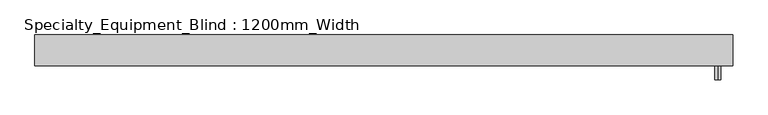
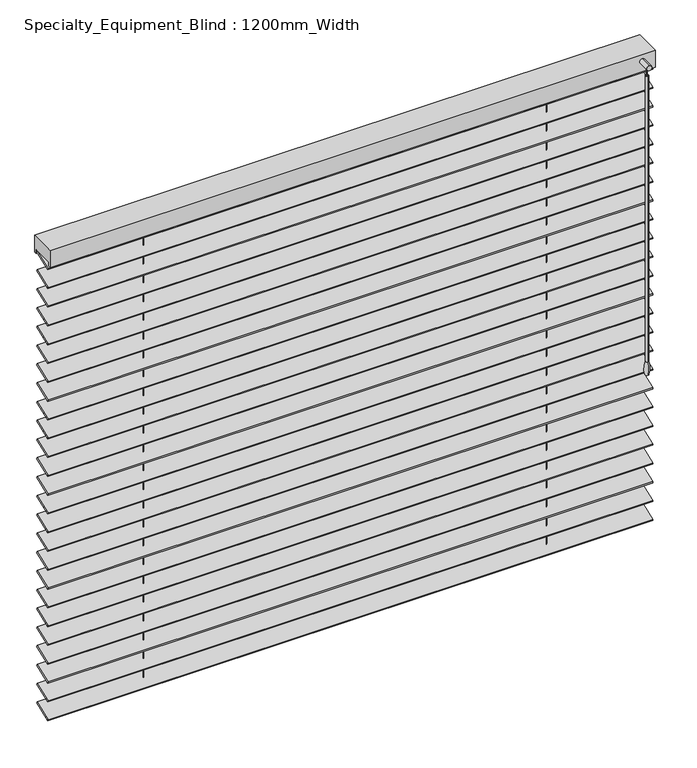
"""IFC4 building model written with IfcOpenShell, lengths in millimetres: proxy geometry, Specialty_Equipment_Blind : 1200mm_Width."""

import ifcopenshell
import ifcopenshell.guid

model = None  # the IFC model being written
_history = None  # IfcOwnerHistory: only IFC2X3 demands one
_inside = {}  # id of a spatial element -> (the spatial element, [elements in it])
_under = {}  # id of a project, library or spatial element -> (it, [spatial elements below it])
_declared = {}  # id of a project -> (the project, [libraries it declares])
_typed = {}  # id of a type object -> (the type object, [elements of that type])
_made_of = {}  # id of a material, layer set ... -> (it, [elements and type objects made of it])


def new_model(schema):
    """Start an empty IFC model of exactly this schema.

    Asked for "IFC4X3", IfcOpenShell would pick the latest addendum, in which some entities
    have other attributes; the version numbers below select the first issue.
    IFC2X3 requires an IfcOwnerHistory on every rooted entity: one is made here for all.
    """
    global model, _history
    if schema == "IFC4X3":
        model = ifcopenshell.file(schema_version=(4, 3, 0, 0))
    else:
        model = ifcopenshell.file(schema=schema)
    _inside.clear()
    _under.clear()
    _declared.clear()
    _typed.clear()
    _made_of.clear()
    _history = None
    if model.schema == "IFC2X3":
        org = make("IfcOrganization", Name="unknown")
        user = make(
            "IfcPersonAndOrganization",
            ThePerson=make("IfcPerson", FamilyName="unknown"),
            TheOrganization=org,
        )
        app = make(
            "IfcApplication",
            ApplicationDeveloper=org,
            Version="unknown",
            ApplicationFullName="unknown",
            ApplicationIdentifier="unknown",
        )
        _history = make(
            "IfcOwnerHistory",
            OwningUser=user,
            OwningApplication=app,
            ChangeAction="ADDED",
            CreationDate=0,
        )
    return model


def make(cls, **values):
    """One entity of the class cls with the attributes given. An attribute that is None is left unset."""
    return model.create_entity(
        cls, **{name: value for name, value in values.items() if value is not None}
    )


def rooted(cls, **values):
    """An entity with a GlobalId (a new one), such as an element, a storey or a relation."""
    return make(cls, GlobalId=ifcopenshell.guid.new(), OwnerHistory=_history, **values)


def si_unit(unit_type, name, prefix=None):
    """IfcSIUnit, for example si_unit("LENGTHUNIT", "METRE", prefix="MILLI")."""
    return make("IfcSIUnit", UnitType=unit_type, Prefix=prefix, Name=name)


def assignment(units):
    """IfcUnitAssignment: the units of a project."""
    return None if units is None else make("IfcUnitAssignment", Units=units)


def point(xyz):
    """IfcCartesianPoint."""
    return None if xyz is None else make("IfcCartesianPoint", Coordinates=xyz)


def direction(xyz):
    """IfcDirection."""
    return None if xyz is None else make("IfcDirection", DirectionRatios=xyz)


def frame(location, z_axis=None, x_axis=None):
    """IfcAxis2Placement3D, a coordinate frame: its origin and axes. An axis left out is left unset."""
    return make(
        "IfcAxis2Placement3D",
        Location=point(location),
        Axis=direction(z_axis),
        RefDirection=direction(x_axis),
    )


def frame_2d(location, x_axis=None):
    """IfcAxis2Placement2D, a coordinate frame in the plane: its origin and x axis."""
    return make(
        "IfcAxis2Placement2D", Location=point(location), RefDirection=direction(x_axis)
    )


def origin():
    """The frame at (0, 0, 0) with its axes left unset."""
    return frame((0.0, 0.0, 0.0))


def place(relative_to, where):
    """IfcLocalPlacement: puts the frame where relative to a parent placement (None: the world)."""
    return make(
        "IfcLocalPlacement", PlacementRelTo=relative_to, RelativePlacement=where
    )


def context(
    kind, dimensions, precision=None, world=None, true_north=None, identifier=None
):
    """IfcGeometricRepresentationContext, for example the 3D "Model" context."""
    return make(
        "IfcGeometricRepresentationContext",
        ContextIdentifier=identifier,
        ContextType=kind,
        CoordinateSpaceDimension=dimensions,
        Precision=precision,
        WorldCoordinateSystem=world,
        TrueNorth=true_north,
    )


def project(units=None, contexts=None):
    """IfcProject with its units and contexts."""
    return rooted(
        "IfcProject",
        Name="project",
        RepresentationContexts=contexts,
        UnitsInContext=assignment(units),
    )


def spatial(cls, under=None, at=None, **own):
    """A site, building, storey or space (cls), placed at a placement, below another one or the project."""
    s = rooted(cls, ObjectPlacement=at, **own)
    if under is not None:
        _under.setdefault(under.id(), (under, []))[1].append(s)
    return s


def polyline(points):
    """IfcPolyline through the points."""
    return make("IfcPolyline", Points=[point(p) for p in points])


def circle_curve(where, radius):
    """IfcCircle in the frame where."""
    return make("IfcCircle", Position=where, Radius=radius)


def ellipse_curve(where, semi_axis1, semi_axis2):
    """IfcEllipse in the frame where."""
    return make(
        "IfcEllipse", Position=where, SemiAxis1=semi_axis1, SemiAxis2=semi_axis2
    )


def trimmed(basis, trim1, trim2, sense, master):
    """IfcTrimmedCurve: the piece of a basis curve between two trims."""
    return make(
        "IfcTrimmedCurve",
        BasisCurve=basis,
        Trim1=trim1,
        Trim2=trim2,
        SenseAgreement=sense,
        MasterRepresentation=master,
    )


def segment(curve, same_sense, transition):
    """IfcCompositeCurveSegment."""
    return make(
        "IfcCompositeCurveSegment",
        Transition=transition,
        SameSense=same_sense,
        ParentCurve=curve,
    )


def composite_curve(segments, self_intersect=None):
    """IfcCompositeCurve: segments joined end to end."""
    return make("IfcCompositeCurve", Segments=segments, SelfIntersect=self_intersect)


def outline(outer, holes=None, kind="AREA"):
    """IfcArbitraryClosedProfileDef: a profile drawn as a closed curve; with holes, ...WithVoids."""
    if holes is None:
        return make("IfcArbitraryClosedProfileDef", ProfileType=kind, OuterCurve=outer)
    return make(
        "IfcArbitraryProfileDefWithVoids",
        ProfileType=kind,
        OuterCurve=outer,
        InnerCurves=holes,
    )


def extrude(swept, where, along, depth):
    """IfcExtrudedAreaSolid: the profile swept, set in the frame where, extruded along a direction by depth."""
    return make(
        "IfcExtrudedAreaSolid",
        SweptArea=swept,
        Position=where,
        ExtrudedDirection=direction(along),
        Depth=depth,
    )


def shape(context_of_items, identifier, shape_type, items):
    """IfcShapeRepresentation: the items that make up one representation, for example the "Body"."""
    return make(
        "IfcShapeRepresentation",
        ContextOfItems=context_of_items,
        RepresentationIdentifier=identifier,
        RepresentationType=shape_type,
        Items=items,
    )


def source(mapping_origin, context_of_items, identifier, shape_type, items):
    """IfcRepresentationMap: a shape defined once, which mapped items show again and again."""
    return make(
        "IfcRepresentationMap",
        MappingOrigin=mapping_origin,
        MappedRepresentation=shape(context_of_items, identifier, shape_type, items),
    )


def transform(
    local_origin,
    x_axis=None,
    y_axis=None,
    z_axis=None,
    scale=None,
    scale2=None,
    scale3=None,
    uniform=True,
):
    """IfcCartesianTransformationOperator3D, or its non-uniform kind. x_axis, y_axis, z_axis: its Axis1, 2, 3."""
    if uniform:
        return make(
            "IfcCartesianTransformationOperator3D",
            Axis1=direction(x_axis),
            Axis2=direction(y_axis),
            LocalOrigin=point(local_origin),
            Scale=scale,
            Axis3=direction(z_axis),
        )
    return make(
        "IfcCartesianTransformationOperator3DnonUniform",
        Axis1=direction(x_axis),
        Axis2=direction(y_axis),
        LocalOrigin=point(local_origin),
        Scale=scale,
        Axis3=direction(z_axis),
        Scale2=scale2,
        Scale3=scale3,
    )


def mapped(mapping_source, mapping_target):
    """IfcMappedItem: shows the shape of a source again, moved by a transform."""
    return make(
        "IfcMappedItem", MappingSource=mapping_source, MappingTarget=mapping_target
    )


def made_of(thing, what):
    """Note that an element or type object is made of a material, layer set ...; save() writes the relation."""
    if what is not None:
        _made_of.setdefault(what.id(), (what, []))[1].append(thing)
    return thing


def element(
    cls,
    number,
    at=None,
    inside=None,
    cuts=None,
    type_object=None,
    material=None,
    context=None,
    identifier="Body",
    shape_type=None,
    held_by="IfcProductDefinitionShape",
    body=None,
    shapes=None,
    **own,
):
    """One element of the class cls, such as IfcWall. Its Tag is "e" and its number.

    at: its placement. inside: the storey or other place that contains it. cuts: it is an
    opening in that element (IfcRelVoidsElement). A single representation is given by context,
    identifier, shape_type and body (its items); several are given by shapes. held_by: the class
    of the entity that holds the representations. save() writes the other relations.
    """
    e = rooted(cls, Tag="e%d" % number, ObjectPlacement=at, **own)
    if body is not None:
        shapes = [shape(context, identifier, shape_type, body)]
    if shapes is not None:
        e.Representation = make(held_by, Representations=shapes)
    if inside is not None:
        _inside.setdefault(inside.id(), (inside, []))[1].append(e)
    if cuts is not None:
        rooted(
            "IfcRelVoidsElement", RelatingBuildingElement=cuts, RelatedOpeningElement=e
        )
    if type_object is not None:
        _typed.setdefault(type_object.id(), (type_object, []))[1].append(e)
    return made_of(e, material)


def aggregate(whole, parts):
    """IfcRelAggregates: a whole, such as a stair, and the parts it consists of."""
    return rooted("IfcRelAggregates", RelatingObject=whole, RelatedObjects=parts)


def save(model, path):
    """Write the relations noted so far, then the file.

    IfcRelAggregates (storeys below a building ...), IfcRelContainedInSpatialStructure (elements
    in a storey), IfcRelDefinesByType, IfcRelAssociatesMaterial and IfcRelDeclares: one each for
    every whole, place, type object, material and project.
    """
    for whole, parts in _under.values():
        aggregate(whole, parts)
    for where, things in _inside.values():
        rooted(
            "IfcRelContainedInSpatialStructure",
            RelatedElements=things,
            RelatingStructure=where,
        )
    for kind, things in _typed.values():
        rooted("IfcRelDefinesByType", RelatedObjects=things, RelatingType=kind)
    for what, things in _made_of.values():
        rooted("IfcRelAssociatesMaterial", RelatedObjects=things, RelatingMaterial=what)
    for by, libraries in _declared.values():
        rooted("IfcRelDeclares", RelatingContext=by, RelatedDefinitions=libraries)
    model.write(path)


def plane_surface(at):
    """IfcPlane: the flat surface through the origin of the frame at, square to its z axis."""
    return make("IfcPlane", Position=at)


def cylinder_surface(at, radius):
    """IfcCylindricalSurface: all points at the distance radius from the z axis of the frame at."""
    return make("IfcCylindricalSurface", Position=at, Radius=radius)


def revolved_surface(curve, axis_point, axis_direction):
    """IfcSurfaceOfRevolution: the curve turned about the line through axis_point along axis_direction."""
    return make(
        "IfcSurfaceOfRevolution",
        SweptCurve=make("IfcArbitraryOpenProfileDef", ProfileType="CURVE", Curve=curve),
        AxisPosition=make("IfcAxis1Placement", Location=point(axis_point), Axis=direction(axis_direction)),
    )


def advanced_brep(points, edges, surfaces, faces):
    """IfcAdvancedBrep: a solid bounded by faces that lie on surfaces and meet in shared edges.

    An edge is (start, end): straight between two places in points (the first is 0);
    or (start, end, curve); or (start, end, curve, False) where it runs against its curve.
    A face is (place in surfaces, loops), or (place, loops, False) where it looks against
    its surface's normal. A loop lists edges by number (the first is 1), with a minus sign
    where the edge is run from its end to its start. The first loop is the outer one.
    """
    corners = [point(p) for p in points]
    vertices = [make("IfcVertexPoint", VertexGeometry=c) for c in corners]
    made = []
    for start, end, *more in edges:
        made.append(
            make(
                "IfcEdgeCurve",
                EdgeStart=vertices[start],
                EdgeEnd=vertices[end],
                EdgeGeometry=more[0] if more else make("IfcPolyline", Points=[corners[start], corners[end]]),
                SameSense=more[1] if len(more) > 1 else True,
            )
        )
    hull = []
    for where, loops, *sense in faces:
        bounds = []
        for j, loop in enumerate(loops):
            ring = [make("IfcOrientedEdge", EdgeElement=made[abs(k) - 1], Orientation=k > 0) for k in loop]
            bounds.append(
                make(
                    "IfcFaceOuterBound" if j == 0 else "IfcFaceBound",
                    Bound=make("IfcEdgeLoop", EdgeList=ring),
                    Orientation=True,
                )
            )
        hull.append(make("IfcAdvancedFace", Bounds=bounds, FaceSurface=surfaces[where], SameSense=sense[0] if sense else True))
    return make("IfcAdvancedBrep", Outer=make("IfcClosedShell", CfsFaces=hull))


def specialty_equipment_blind_1200mm_width_23c077ca(model_context):
    return source(origin(), model_context, "Body", "SolidModel", [
        extrude(outline(polyline([(0.0, -40.0), (0.0, 0.0), (1180.0, 0.0), (1180.0, -40.0), (0.0, -40.0)])), frame((-439.5079376, 65.0532351, 2040.2125618), z_axis=(0.0, -0.3420201433256684, 0.9396926207859085), x_axis=(1.0, 0.0, 0.0)), (0.0, 0.0, 1.0), 3.0625345),
        extrude(outline(polyline([(0.0, -40.0), (0.0, 0.0), (1180.0, 0.0), (1180.0, -40.0), (0.0, -40.0)])), frame((-439.5079376, 65.0532351, 2001.4625618), z_axis=(0.0, -0.3420201433256684, 0.9396926207859085), x_axis=(1.0, 0.0, 0.0)), (0.0, 0.0, 1.0), 3.0625345),
        extrude(outline(polyline([(0.0, -40.0), (0.0, 0.0), (1180.0, 0.0), (1180.0, -40.0), (0.0, -40.0)])), frame((-439.5079376, 65.0532351, 1962.7125618), z_axis=(0.0, -0.3420201433256684, 0.9396926207859085), x_axis=(1.0, 0.0, 0.0)), (0.0, 0.0, 1.0), 3.0625345),
        extrude(outline(polyline([(0.0, -40.0), (0.0, 0.0), (1180.0, 0.0), (1180.0, -40.0), (0.0, -40.0)])), frame((-439.5079376, 65.0532351, 1923.9625618), z_axis=(0.0, -0.3420201433256684, 0.9396926207859085), x_axis=(1.0, 0.0, 0.0)), (0.0, 0.0, 1.0), 3.0625345),
        extrude(outline(polyline([(0.0, -40.0), (0.0, 0.0), (1180.0, 0.0), (1180.0, -40.0), (0.0, -40.0)])), frame((-439.5079376, 65.0532351, 1885.2125618), z_axis=(0.0, -0.3420201433256684, 0.9396926207859085), x_axis=(1.0, 0.0, 0.0)), (0.0, 0.0, 1.0), 3.0625345),
        extrude(outline(polyline([(0.0, -40.0), (0.0, 0.0), (1180.0, 0.0), (1180.0, -40.0), (0.0, -40.0)])), frame((-439.5079376, 65.0532351, 1846.4625618), z_axis=(0.0, -0.3420201433256684, 0.9396926207859085), x_axis=(1.0, 0.0, 0.0)), (0.0, 0.0, 1.0), 3.0625345),
        extrude(outline(polyline([(0.0, -40.0), (0.0, 0.0), (1180.0, 0.0), (1180.0, -40.0), (0.0, -40.0)])), frame((-439.5079376, 65.0532351, 1807.7125618), z_axis=(0.0, -0.3420201433256684, 0.9396926207859085), x_axis=(1.0, 0.0, 0.0)), (0.0, 0.0, 1.0), 3.0625345),
        extrude(outline(polyline([(0.0, -40.0), (0.0, 0.0), (1180.0, 0.0), (1180.0, -40.0), (0.0, -40.0)])), frame((-439.5079376, 65.0532351, 1768.9625618), z_axis=(0.0, -0.3420201433256684, 0.9396926207859085), x_axis=(1.0, 0.0, 0.0)), (0.0, 0.0, 1.0), 3.0625345),
        extrude(outline(polyline([(0.0, -40.0), (0.0, 0.0), (1180.0, 0.0), (1180.0, -40.0), (0.0, -40.0)])), frame((-439.5079376, 65.0532351, 1730.2125618), z_axis=(0.0, -0.3420201433256684, 0.9396926207859085), x_axis=(1.0, 0.0, 0.0)), (0.0, 0.0, 1.0), 3.0625345),
        extrude(outline(polyline([(0.0, -40.0), (0.0, 0.0), (1180.0, 0.0), (1180.0, -40.0), (0.0, -40.0)])), frame((-439.5079376, 65.0532351, 1691.4625618), z_axis=(0.0, -0.3420201433256684, 0.9396926207859085), x_axis=(1.0, 0.0, 0.0)), (0.0, 0.0, 1.0), 3.0625345),
        extrude(outline(polyline([(0.0, -40.0), (0.0, 0.0), (1180.0, 0.0), (1180.0, -40.0), (0.0, -40.0)])), frame((-439.5079376, 65.0532351, 1652.7125618), z_axis=(0.0, -0.3420201433256684, 0.9396926207859085), x_axis=(1.0, 0.0, 0.0)), (0.0, 0.0, 1.0), 3.0625345),
        extrude(outline(polyline([(0.0, -40.0), (0.0, 0.0), (1180.0, 0.0), (1180.0, -40.0), (0.0, -40.0)])), frame((-439.5079376, 65.0532351, 1613.9625618), z_axis=(0.0, -0.3420201433256684, 0.9396926207859085), x_axis=(1.0, 0.0, 0.0)), (0.0, 0.0, 1.0), 3.0625345),
        extrude(outline(polyline([(0.0, -40.0), (0.0, 0.0), (1180.0, 0.0), (1180.0, -40.0), (0.0, -40.0)])), frame((-439.5079376, 65.0532351, 1575.2125618), z_axis=(0.0, -0.3420201433256684, 0.9396926207859085), x_axis=(1.0, 0.0, 0.0)), (0.0, 0.0, 1.0), 3.0625345),
        extrude(outline(polyline([(0.0, -40.0), (0.0, 0.0), (1180.0, 0.0), (1180.0, -40.0), (0.0, -40.0)])), frame((-439.5079376, 65.0532351, 1536.4625618), z_axis=(0.0, -0.3420201433256684, 0.9396926207859085), x_axis=(1.0, 0.0, 0.0)), (0.0, 0.0, 1.0), 3.0625345),
        extrude(outline(polyline([(0.0, -40.0), (0.0, 0.0), (1180.0, 0.0), (1180.0, -40.0), (0.0, -40.0)])), frame((-439.5079376, 65.0532351, 1497.7125618), z_axis=(0.0, -0.3420201433256684, 0.9396926207859085), x_axis=(1.0, 0.0, 0.0)), (0.0, 0.0, 1.0), 3.0625345),
        extrude(outline(polyline([(0.0, -40.0), (0.0, 0.0), (1180.0, 0.0), (1180.0, -40.0), (0.0, -40.0)])), frame((-439.5079376, 65.0532351, 1458.9625618), z_axis=(0.0, -0.3420201433256684, 0.9396926207859085), x_axis=(1.0, 0.0, 0.0)), (0.0, 0.0, 1.0), 3.0625345),
        extrude(outline(polyline([(0.0, -40.0), (0.0, 0.0), (1180.0, 0.0), (1180.0, -40.0), (0.0, -40.0)])), frame((-439.5079376, 65.0532351, 1420.2125618), z_axis=(0.0, -0.3420201433256684, 0.9396926207859085), x_axis=(1.0, 0.0, 0.0)), (0.0, 0.0, 1.0), 3.0625345),
        extrude(outline(polyline([(0.0, -40.0), (0.0, 0.0), (1180.0, 0.0), (1180.0, -40.0), (0.0, -40.0)])), frame((-439.5079376, 65.0532351, 1381.4625618), z_axis=(0.0, -0.3420201433256684, 0.9396926207859085), x_axis=(1.0, 0.0, 0.0)), (0.0, 0.0, 1.0), 3.0625345),
        extrude(outline(polyline([(0.0, -40.0), (0.0, 0.0), (1180.0, 0.0), (1180.0, -40.0), (0.0, -40.0)])), frame((-439.5079376, 65.0532351, 1342.7125618), z_axis=(0.0, -0.3420201433256684, 0.9396926207859085), x_axis=(1.0, 0.0, 0.0)), (0.0, 0.0, 1.0), 3.0625345),
        extrude(outline(polyline([(0.0, -40.0), (0.0, 0.0), (1180.0, 0.0), (1180.0, -40.0), (0.0, -40.0)])), frame((-439.5079376, 65.0532351, 1303.9625618), z_axis=(0.0, -0.3420201433256684, 0.9396926207859085), x_axis=(1.0, 0.0, 0.0)), (0.0, 0.0, 1.0), 3.0625345),
        extrude(outline(polyline([(0.0, -40.0), (0.0, 0.0), (1180.0, 0.0), (1180.0, -40.0), (0.0, -40.0)])), frame((-439.5079376, 65.0532351, 1265.2125618), z_axis=(0.0, -0.3420201433256684, 0.9396926207859085), x_axis=(1.0, 0.0, 0.0)), (0.0, 0.0, 1.0), 3.0625345),
        extrude(outline(polyline([(0.0, -40.0), (0.0, 0.0), (1180.0, 0.0), (1180.0, -40.0), (0.0, -40.0)])), frame((-439.5079376, 65.0532351, 1226.4625618), z_axis=(0.0, -0.3420201433256684, 0.9396926207859085), x_axis=(1.0, 0.0, 0.0)), (0.0, 0.0, 1.0), 3.0625345),
        extrude(outline(polyline([(0.0, -40.0), (0.0, 0.0), (1180.0, 0.0), (1180.0, -40.0), (0.0, -40.0)])), frame((-439.5079376, 65.0532351, 1187.7125618), z_axis=(0.0, -0.3420201433256684, 0.9396926207859085), x_axis=(1.0, 0.0, 0.0)), (0.0, 0.0, 1.0), 3.0625345),
        extrude(outline(polyline([(0.0, -40.0), (0.0, 0.0), (1180.0, 0.0), (1180.0, -40.0), (0.0, -40.0)])), frame((-439.5079376, 65.0532351, 2078.9625618), z_axis=(0.0, -0.3420201433256684, 0.9396926207859085), x_axis=(1.0, 0.0, 0.0)), (0.0, 0.0, 1.0), 3.0625345),
        extrude(outline(polyline([(0.0, -40.0), (0.0, 0.0), (1180.0, 0.0), (1180.0, -40.0), (0.0, -40.0)])), frame((-439.5079376, 65.0532351, 1148.9625618), z_axis=(0.0, -0.3420201433256684, 0.9396926207859085), x_axis=(1.0, 0.0, 0.0)), (0.0, 0.0, 1.0), 3.0625345),
        extrude(outline(composite_curve([segment(trimmed(circle_curve(frame_2d((-242.8412709, 45.2119342)), 0.5), [point((-243.3412709, 45.2119342))], [point((-242.3412709, 45.2119342))], False, "CARTESIAN"), True, "CONTINUOUS"), segment(trimmed(circle_curve(frame_2d((-242.8412709, 45.2119342)), 0.5), [point((-242.3412709, 45.2119342))], [point((-243.3412709, 45.2119342))], False, "CARTESIAN"), True, "CONTINUOUS")], self_intersect=False)), frame((0.0, 0.0, 1130.0), z_axis=(0.0, 0.0, 1.0), x_axis=(1.0, 0.0, 0.0)), (0.0, 0.0, 1.0), 953.2448883),
        extrude(outline(composite_curve([segment(trimmed(circle_curve(frame_2d((543.8253958, 45.2119342)), 0.5), [point((543.3253958, 45.2119342))], [point((544.3253958, 45.2119342))], False, "CARTESIAN"), True, "CONTINUOUS"), segment(trimmed(circle_curve(frame_2d((543.8253958, 45.2119342)), 0.5), [point((544.3253958, 45.2119342))], [point((543.3253958, 45.2119342))], False, "CARTESIAN"), True, "CONTINUOUS")], self_intersect=False)), frame((0.0, 0.0, 1130.0), z_axis=(0.0, 0.0, 1.0), x_axis=(1.0, 0.0, 0.0)), (0.0, 0.0, 1.0), 953.2448883),
        advanced_brep(
        [(715.4920624, 4.7248495, 2091.3243671), (715.4920624, 2.7248495, 2091.3243671), (715.4920624, 3.7248495, 2091.3243671), (715.4920624, 4.7248495, 2076.3243671), (715.4920624, 2.7248495, 2076.3243671), (715.4920624, 6.7248495, 2076.3243671), (715.4920624, 0.7248495, 2076.3243671), (715.4920624, 6.7248495, 1486.909931), (715.4920624, 0.7248495, 1486.909931), (715.4920624, 7.2513368, 1460.0), (715.4920624, 0.1983622, 1460.0), (715.4920624, 3.7248495, 1460.0)],
        [
            (0, 1, circle_curve(frame((715.4920624, 3.7248495, 2091.3243671), z_axis=(0.0, 0.0, 1.0), x_axis=(0.0, -1.0, 0.0)), 1.0)),
            (1, 2),
            (2, 0),
            (1, 0, circle_curve(frame((715.4920624, 3.7248495, 2091.3243671), z_axis=(0.0, 0.0, 1.0), x_axis=(0.0, -1.0, 0.0)), 1.0)),
            (3, 4, circle_curve(frame((715.4920624, 3.7248495, 2076.3243671), z_axis=(0.0, 0.0, 1.0), x_axis=(0.0, -1.0, 0.0)), 1.0)),
            (4, 1),
            (0, 3),
            (4, 3, circle_curve(frame((715.4920624, 3.7248495, 2076.3243671), z_axis=(0.0, 0.0, 1.0), x_axis=(0.0, -1.0, 0.0)), 1.0)),
            (5, 6, circle_curve(frame((715.4920624, 3.7248495, 2076.3243671), z_axis=(0.0, 0.0, 1.0), x_axis=(0.0, -1.0, 0.0)), 3.0)),
            (6, 4),
            (3, 5),
            (6, 5, circle_curve(frame((715.4920624, 3.7248495, 2076.3243671), z_axis=(0.0, 0.0, 1.0), x_axis=(0.0, -1.0, 0.0)), 3.0)),
            (7, 8, circle_curve(frame((715.4920624, 3.7248495, 1486.909931), z_axis=(0.0, 0.0, 1.0), x_axis=(0.0, -1.0, 0.0)), 3.0)),
            (8, 6),
            (5, 7),
            (8, 7, circle_curve(frame((715.4920624, 3.7248495, 1486.909931), z_axis=(0.0, 0.0, 1.0), x_axis=(0.0, -1.0, 0.0)), 3.0)),
            (9, 10, circle_curve(frame((715.4920624, 3.7248495, 1460.0), z_axis=(0.0, 0.0, 1.0), x_axis=(0.0, -1.0, 0.0)), 3.5264873)),
            (10, 8, circle_curve(frame((715.4920624, 49.2720063, 1472.5), z_axis=(-1.0, 0.0, 0.0), x_axis=(0.0, 1.0, 0.0)), 50.6406214)),
            (7, 9, circle_curve(frame((715.4920624, -41.8223072, 1472.5), z_axis=(-1.0, 0.0, 0.0), x_axis=(0.0, -1.0, 0.0)), 50.6406214)),
            (10, 9, circle_curve(frame((715.4920624, 3.7248495, 1460.0), z_axis=(0.0, 0.0, 1.0), x_axis=(0.0, -1.0, 0.0)), 3.5264873)),
            (11, 10),
            (9, 11),
        ],
        [
            plane_surface(frame((715.4920624, 3.7248495, 2091.3243671), z_axis=(0.0, 0.0, 1.0), x_axis=(0.0, -1.0, 0.0))),
            cylinder_surface(frame((715.4920624, 3.7248495, 1191.3243671), z_axis=(0.0, 0.0, -1.0), x_axis=(0.0, -1.0, 0.0)), 1.0),
            plane_surface(frame((715.4920624, 3.7248495, 2076.3243671), z_axis=(0.0, 0.0, 1.0), x_axis=(0.0, -1.0, 0.0))),
            cylinder_surface(frame((715.4920624, 3.7248495, 1191.3243671), z_axis=(0.0, 0.0, -1.0), x_axis=(0.0, -1.0, 0.0)), 3.0),
            revolved_surface(trimmed(ellipse_curve(frame((715.4920624, 49.2720063, 1472.5), z_axis=(1.0, 0.0, 0.0), x_axis=(0.0, 1.0, 0.0)), 50.6406214, 50.6406214), [point((715.4920624, 0.7248495, 1486.909931))], [point((715.4920624, 0.1983622, 1460.0))], True, "CARTESIAN"), (715.4920624, 3.7248495, 1191.3243671), (0.0, 0.0, -1.0)),
            plane_surface(frame((715.4920624, 3.7248495, 1460.0), z_axis=(0.0, 0.0, -1.0), x_axis=(0.0, -1.0, 0.0))),
        ],
        [
            (0, [[1, 2, 3]]),
            (0, [[4, -3, -2]]),
            (1, [[5, 6, -1, 7]]),
            (1, [[8, -7, -4, -6]]),
            (2, [[9, 10, -5, 11]]),
            (2, [[12, -11, -8, -10]]),
            (3, [[13, 14, -9, 15]]),
            (3, [[16, -15, -12, -14]]),
            (4, [[17, 18, -13, 19]]),
            (4, [[20, -19, -16, -18]]),
            (5, [[21, -17, 22]]),
            (5, [[-22, -20, -21]]),
        ],
    ),
        extrude(outline(composite_curve([segment(trimmed(circle_curve(frame_2d((2095.9171213, 715.4920624)), 5.0), [point((2100.9171213, 715.4920624))], [point((2090.9171213, 715.4920624))], False, "CARTESIAN"), True, "CONTINUOUS"), segment(trimmed(circle_curve(frame_2d((2095.9171213, 715.4920624)), 5.0), [point((2090.9171213, 715.4920624))], [point((2100.9171213, 715.4920624))], False, "CARTESIAN"), True, "CONTINUOUS")], self_intersect=False)), frame((0.0, -4.4512463, 0.0), z_axis=(0.0, 1.0, 0.0), x_axis=(0.0, 0.0, 1.0)), (0.0, 0.0, 1.0), 23.7809602),
        extrude(outline(polyline([(19.329714, 2110.0), (71.0941545, 2110.0), (71.0941545, 2075.0), (66.0941545, 2075.0), (66.0941545, 2083.2448883), (24.329714, 2083.2448883), (24.329714, 2075.0), (19.329714, 2075.0), (19.329714, 2110.0)])), frame((-439.5079376, 0.0, 0.0), z_axis=(1.0, 0.0, 0.0), x_axis=(0.0, 1.0, 0.0)), (0.0, 0.0, 1.0), 1180.0),
    ])


if __name__ == "__main__":
    model = new_model("IFC4")
    model_context = context("Model", 3, world=origin())
    ifc_project = project(units=[si_unit("LENGTHUNIT", "METRE", prefix="MILLI")], contexts=[model_context])
    site = spatial("IfcSite", under=ifc_project)
    building = spatial("IfcBuilding", under=site)
    placement = place(None, origin())
    specialty_equipment_blind_1200mm_width_shape = specialty_equipment_blind_1200mm_width_23c077ca(model_context)
    element("IfcBuildingElementProxy", 1, Name="Specialty_Equipment_Blind : 1200mm_Width", ObjectType="Specialty_Equipment_Blind : 1200mm_Width", at=placement, inside=building, context=model_context, shape_type="MappedRepresentation", body=[
        mapped(specialty_equipment_blind_1200mm_width_shape, transform((0.0, 0.0, 0.0), x_axis=(1.0, 0.0, 0.0), y_axis=(0.0, 1.0, 0.0), z_axis=(0.0, 0.0, 1.0))),
    ])
    save(model, "model.ifc")

# Revit data of these elements
# Type "Specialty_Equipment_Blind : 1200mm_Width"
#   Keynote = "N10/240"
#   Opening Width = 1200 mm
#   End Offset = 10 mm
#   Blind Length = 1180 mm
#   Blind Fixing Height = 2110 mm
#   Blind Depth = 980 mm
#   Blind Angle = 20.00°
#   Blade Depth = 40 mm
#   No of Blades = 25
#   Material Blind = Wood - Birch
#   Default Elevation = 0
# Element 1 (IfcBuildingElementProxy, "Specialty_Equipment_Blind : 1200mm_Width")
#   Materials on its faces: "Wood - Birch"
# Materials
#   "Wood - Birch": class "Wood", colour RGB 224 178 126, transparency 0
